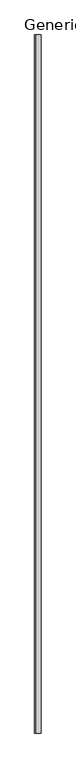
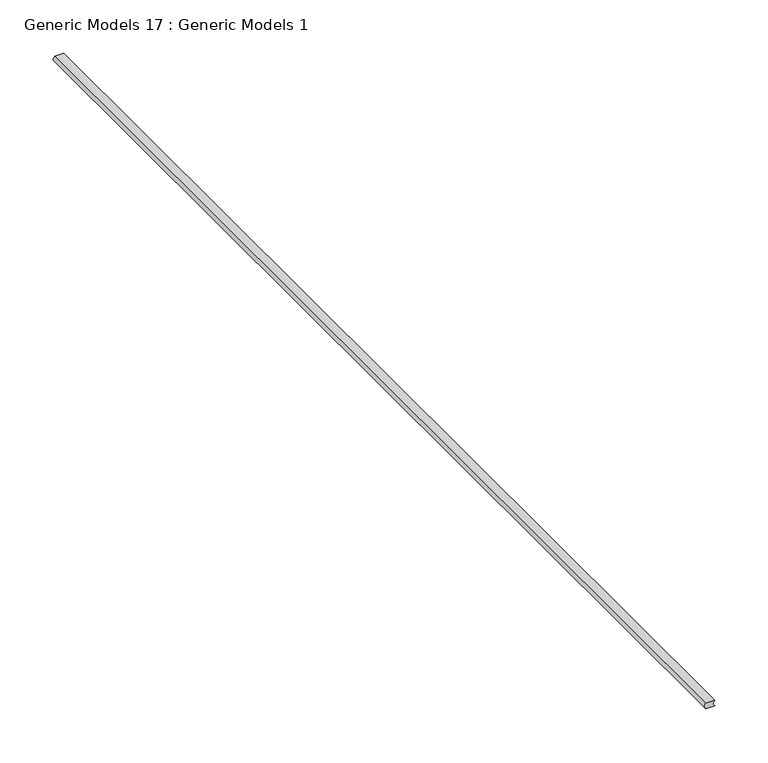
"""IFC4 building model written with IfcOpenShell, lengths in millimetres: proxy geometry, Generic Models 17 : Generic Models 1."""

import ifcopenshell
import ifcopenshell.guid

model = None  # the IFC model being written
_history = None  # IfcOwnerHistory: only IFC2X3 demands one
_inside = {}  # id of a spatial element -> (the spatial element, [elements in it])
_under = {}  # id of a project, library or spatial element -> (it, [spatial elements below it])
_declared = {}  # id of a project -> (the project, [libraries it declares])
_typed = {}  # id of a type object -> (the type object, [elements of that type])
_made_of = {}  # id of a material, layer set ... -> (it, [elements and type objects made of it])


def new_model(schema):
    """Start an empty IFC model of exactly this schema.

    Asked for "IFC4X3", IfcOpenShell would pick the latest addendum, in which some entities
    have other attributes; the version numbers below select the first issue.
    IFC2X3 requires an IfcOwnerHistory on every rooted entity: one is made here for all.
    """
    global model, _history
    if schema == "IFC4X3":
        model = ifcopenshell.file(schema_version=(4, 3, 0, 0))
    else:
        model = ifcopenshell.file(schema=schema)
    _inside.clear()
    _under.clear()
    _declared.clear()
    _typed.clear()
    _made_of.clear()
    _history = None
    if model.schema == "IFC2X3":
        org = make("IfcOrganization", Name="unknown")
        user = make(
            "IfcPersonAndOrganization",
            ThePerson=make("IfcPerson", FamilyName="unknown"),
            TheOrganization=org,
        )
        app = make(
            "IfcApplication",
            ApplicationDeveloper=org,
            Version="unknown",
            ApplicationFullName="unknown",
            ApplicationIdentifier="unknown",
        )
        _history = make(
            "IfcOwnerHistory",
            OwningUser=user,
            OwningApplication=app,
            ChangeAction="ADDED",
            CreationDate=0,
        )
    return model


def make(cls, **values):
    """One entity of the class cls with the attributes given. An attribute that is None is left unset."""
    return model.create_entity(
        cls, **{name: value for name, value in values.items() if value is not None}
    )


def rooted(cls, **values):
    """An entity with a GlobalId (a new one), such as an element, a storey or a relation."""
    return make(cls, GlobalId=ifcopenshell.guid.new(), OwnerHistory=_history, **values)


def si_unit(unit_type, name, prefix=None):
    """IfcSIUnit, for example si_unit("LENGTHUNIT", "METRE", prefix="MILLI")."""
    return make("IfcSIUnit", UnitType=unit_type, Prefix=prefix, Name=name)


def assignment(units):
    """IfcUnitAssignment: the units of a project."""
    return None if units is None else make("IfcUnitAssignment", Units=units)


def point(xyz):
    """IfcCartesianPoint."""
    return None if xyz is None else make("IfcCartesianPoint", Coordinates=xyz)


def direction(xyz):
    """IfcDirection."""
    return None if xyz is None else make("IfcDirection", DirectionRatios=xyz)


def frame(location, z_axis=None, x_axis=None):
    """IfcAxis2Placement3D, a coordinate frame: its origin and axes. An axis left out is left unset."""
    return make(
        "IfcAxis2Placement3D",
        Location=point(location),
        Axis=direction(z_axis),
        RefDirection=direction(x_axis),
    )


def frame_2d(location, x_axis=None):
    """IfcAxis2Placement2D, a coordinate frame in the plane: its origin and x axis."""
    return make(
        "IfcAxis2Placement2D", Location=point(location), RefDirection=direction(x_axis)
    )


def origin():
    """The frame at (0, 0, 0) with its axes left unset."""
    return frame((0.0, 0.0, 0.0))


def place(relative_to, where):
    """IfcLocalPlacement: puts the frame where relative to a parent placement (None: the world)."""
    return make(
        "IfcLocalPlacement", PlacementRelTo=relative_to, RelativePlacement=where
    )


def context(
    kind, dimensions, precision=None, world=None, true_north=None, identifier=None
):
    """IfcGeometricRepresentationContext, for example the 3D "Model" context."""
    return make(
        "IfcGeometricRepresentationContext",
        ContextIdentifier=identifier,
        ContextType=kind,
        CoordinateSpaceDimension=dimensions,
        Precision=precision,
        WorldCoordinateSystem=world,
        TrueNorth=true_north,
    )


def project(units=None, contexts=None):
    """IfcProject with its units and contexts."""
    return rooted(
        "IfcProject",
        Name="project",
        RepresentationContexts=contexts,
        UnitsInContext=assignment(units),
    )


def spatial(cls, under=None, at=None, **own):
    """A site, building, storey or space (cls), placed at a placement, below another one or the project."""
    s = rooted(cls, ObjectPlacement=at, **own)
    if under is not None:
        _under.setdefault(under.id(), (under, []))[1].append(s)
    return s


def polyline(points):
    """IfcPolyline through the points."""
    return make("IfcPolyline", Points=[point(p) for p in points])


def circle_curve(where, radius):
    """IfcCircle in the frame where."""
    return make("IfcCircle", Position=where, Radius=radius)


def trimmed(basis, trim1, trim2, sense, master):
    """IfcTrimmedCurve: the piece of a basis curve between two trims."""
    return make(
        "IfcTrimmedCurve",
        BasisCurve=basis,
        Trim1=trim1,
        Trim2=trim2,
        SenseAgreement=sense,
        MasterRepresentation=master,
    )


def segment(curve, same_sense, transition):
    """IfcCompositeCurveSegment."""
    return make(
        "IfcCompositeCurveSegment",
        Transition=transition,
        SameSense=same_sense,
        ParentCurve=curve,
    )


def composite_curve(segments, self_intersect=None):
    """IfcCompositeCurve: segments joined end to end."""
    return make("IfcCompositeCurve", Segments=segments, SelfIntersect=self_intersect)


def outline(outer, holes=None, kind="AREA"):
    """IfcArbitraryClosedProfileDef: a profile drawn as a closed curve; with holes, ...WithVoids."""
    if holes is None:
        return make("IfcArbitraryClosedProfileDef", ProfileType=kind, OuterCurve=outer)
    return make(
        "IfcArbitraryProfileDefWithVoids",
        ProfileType=kind,
        OuterCurve=outer,
        InnerCurves=holes,
    )


def extrude(swept, where, along, depth):
    """IfcExtrudedAreaSolid: the profile swept, set in the frame where, extruded along a direction by depth."""
    return make(
        "IfcExtrudedAreaSolid",
        SweptArea=swept,
        Position=where,
        ExtrudedDirection=direction(along),
        Depth=depth,
    )


def shape(context_of_items, identifier, shape_type, items):
    """IfcShapeRepresentation: the items that make up one representation, for example the "Body"."""
    return make(
        "IfcShapeRepresentation",
        ContextOfItems=context_of_items,
        RepresentationIdentifier=identifier,
        RepresentationType=shape_type,
        Items=items,
    )


def source(mapping_origin, context_of_items, identifier, shape_type, items):
    """IfcRepresentationMap: a shape defined once, which mapped items show again and again."""
    return make(
        "IfcRepresentationMap",
        MappingOrigin=mapping_origin,
        MappedRepresentation=shape(context_of_items, identifier, shape_type, items),
    )


def transform(
    local_origin,
    x_axis=None,
    y_axis=None,
    z_axis=None,
    scale=None,
    scale2=None,
    scale3=None,
    uniform=True,
):
    """IfcCartesianTransformationOperator3D, or its non-uniform kind. x_axis, y_axis, z_axis: its Axis1, 2, 3."""
    if uniform:
        return make(
            "IfcCartesianTransformationOperator3D",
            Axis1=direction(x_axis),
            Axis2=direction(y_axis),
            LocalOrigin=point(local_origin),
            Scale=scale,
            Axis3=direction(z_axis),
        )
    return make(
        "IfcCartesianTransformationOperator3DnonUniform",
        Axis1=direction(x_axis),
        Axis2=direction(y_axis),
        LocalOrigin=point(local_origin),
        Scale=scale,
        Axis3=direction(z_axis),
        Scale2=scale2,
        Scale3=scale3,
    )


def mapped(mapping_source, mapping_target):
    """IfcMappedItem: shows the shape of a source again, moved by a transform."""
    return make(
        "IfcMappedItem", MappingSource=mapping_source, MappingTarget=mapping_target
    )


def made_of(thing, what):
    """Note that an element or type object is made of a material, layer set ...; save() writes the relation."""
    if what is not None:
        _made_of.setdefault(what.id(), (what, []))[1].append(thing)
    return thing


def element(
    cls,
    number,
    at=None,
    inside=None,
    cuts=None,
    type_object=None,
    material=None,
    context=None,
    identifier="Body",
    shape_type=None,
    held_by="IfcProductDefinitionShape",
    body=None,
    shapes=None,
    **own,
):
    """One element of the class cls, such as IfcWall. Its Tag is "e" and its number.

    at: its placement. inside: the storey or other place that contains it. cuts: it is an
    opening in that element (IfcRelVoidsElement). A single representation is given by context,
    identifier, shape_type and body (its items); several are given by shapes. held_by: the class
    of the entity that holds the representations. save() writes the other relations.
    """
    e = rooted(cls, Tag="e%d" % number, ObjectPlacement=at, **own)
    if body is not None:
        shapes = [shape(context, identifier, shape_type, body)]
    if shapes is not None:
        e.Representation = make(held_by, Representations=shapes)
    if inside is not None:
        _inside.setdefault(inside.id(), (inside, []))[1].append(e)
    if cuts is not None:
        rooted(
            "IfcRelVoidsElement", RelatingBuildingElement=cuts, RelatedOpeningElement=e
        )
    if type_object is not None:
        _typed.setdefault(type_object.id(), (type_object, []))[1].append(e)
    return made_of(e, material)


def aggregate(whole, parts):
    """IfcRelAggregates: a whole, such as a stair, and the parts it consists of."""
    return rooted("IfcRelAggregates", RelatingObject=whole, RelatedObjects=parts)


def save(model, path):
    """Write the relations noted so far, then the file.

    IfcRelAggregates (storeys below a building ...), IfcRelContainedInSpatialStructure (elements
    in a storey), IfcRelDefinesByType, IfcRelAssociatesMaterial and IfcRelDeclares: one each for
    every whole, place, type object, material and project.
    """
    for whole, parts in _under.values():
        aggregate(whole, parts)
    for where, things in _inside.values():
        rooted(
            "IfcRelContainedInSpatialStructure",
            RelatedElements=things,
            RelatingStructure=where,
        )
    for kind, things in _typed.values():
        rooted("IfcRelDefinesByType", RelatedObjects=things, RelatingType=kind)
    for what, things in _made_of.values():
        rooted("IfcRelAssociatesMaterial", RelatedObjects=things, RelatingMaterial=what)
    for by, libraries in _declared.values():
        rooted("IfcRelDeclares", RelatingContext=by, RelatedDefinitions=libraries)
    model.write(path)


def generic_models_17_generic_models_1_5a74d62d(model_context):
    return source(origin(), model_context, "Body", "SweptSolid", [
        extrude(outline(composite_curve([segment(trimmed(circle_curve(frame_2d((3.175, 49802.7897405)), 4.3100275), [point((0.0, 49799.875))], [point((6.35, 49799.875))], True, "CARTESIAN"), True, "CONTINUOUS"), segment(polyline([(6.35, 49799.875), (6.35, 49790.35)]), True, "CONTINUOUS"), segment(trimmed(circle_curve(frame_2d((3.175, 49793.2647405)), 4.3100275), [point((6.35, 49790.35))], [point((0.0, 49790.35))], False, "CARTESIAN"), True, "CONTINUOUS"), segment(polyline([(0.0, 49790.35), (0.0, 49799.875)]), True, "CONTINUOUS")], self_intersect=False)), frame((0.0, 0.0, 0.0), z_axis=(0.0, 1.0, 0.0), x_axis=(0.0, 0.0, 1.0)), (0.0, 0.0, 1.0), 1219.2),
    ])


if __name__ == "__main__":
    model = new_model("IFC4")
    model_context = context("Model", 3, world=origin())
    ifc_project = project(units=[si_unit("LENGTHUNIT", "METRE", prefix="MILLI")], contexts=[model_context])
    site = spatial("IfcSite", under=ifc_project)
    building = spatial("IfcBuilding", under=site)
    placement = place(None, origin())
    generic_models_17_generic_models_1_shape = generic_models_17_generic_models_1_5a74d62d(model_context)
    element("IfcBuildingElementProxy", 1, Name="Generic Models 17 : Generic Models 1", ObjectType="Generic Models 17 : Generic Models 1", at=placement, inside=building, context=model_context, shape_type="MappedRepresentation", body=[
        mapped(generic_models_17_generic_models_1_shape, transform((0.0, 0.0, 0.0), x_axis=(1.0, 0.0, 0.0), y_axis=(0.0, 1.0, 0.0), z_axis=(0.0, 0.0, 1.0))),
    ])
    save(model, "model.ifc")

# Revit data of these elements
# Element 1 (IfcBuildingElementProxy, "Generic Models 17 : Generic Models 1")
#   Materials on its faces: "ACOUSTICAL SEALANT"
# Materials
#   "ACOUSTICAL SEALANT": class "Unassigned", colour RGB 120 120 120, transparency 0, Cost = 0
